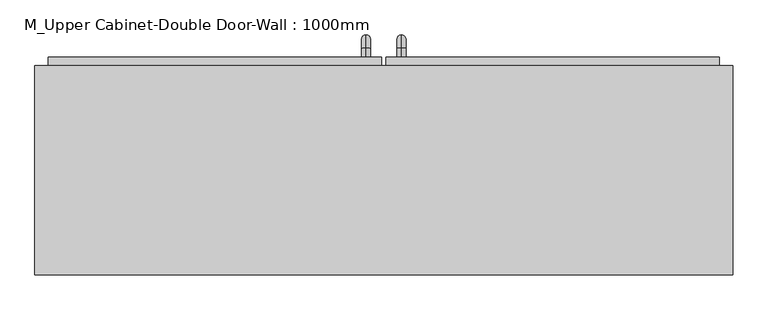
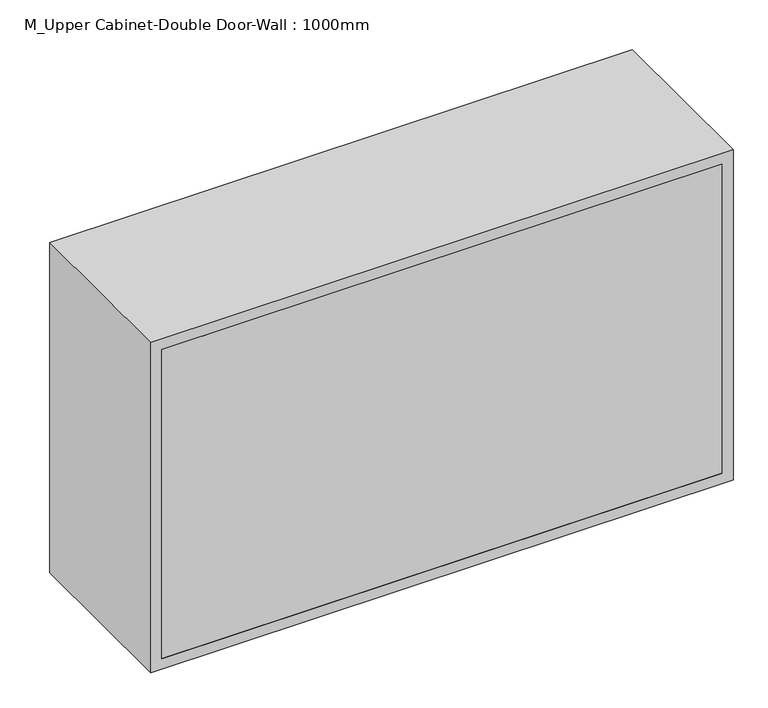
"""IFC4 building model written with IfcOpenShell, lengths in millimetres: furniture geometry, M_Upper Cabinet-Double Door-Wall : 1000mm."""

from ifc_helpers import new_model, si_unit, point, frame, origin, place, context, project, spatial, polyline, circle_curve, ellipse_curve, trimmed, outline, extrude, source, transform, mapped, element, save
from ifc_brep_helpers import plane_surface, cylinder_surface, revolved_surface, advanced_brep


def m_upper_cabinet_double_door_wall_1000mm_a8185405(model_context):
    return source(origin(), model_context, "Body", "SolidModel", [
        extrude(outline(polyline([(2000.0, -470.2288372), (1400.0, -470.2288372), (1400.0, 529.7711628), (2000.0, 529.7711628), (2000.0, -470.2288372)]), holes=[polyline([(1980.95, -451.1788372), (1980.95, 510.7211628), (1419.05, 510.7211628), (1419.05, -451.1788372), (1980.95, -451.1788372)])]), frame((0.0, 174.5, 0.0), z_axis=(0.0, 1.0, 0.0), x_axis=(0.0, 0.0, 1.0)), (0.0, 0.0, 1.0), 300.0),
        extrude(outline(polyline([(510.7211628, 174.5), (-451.1788372, 174.5), (-451.1788372, 193.55), (510.7211628, 193.55), (510.7211628, 174.5)])), frame((0.0, 0.0, 1419.05), z_axis=(0.0, 0.0, 1.0), x_axis=(1.0, 0.0, 0.0)), (0.0, 0.0, 1.0), 561.9),
        extrude(outline(polyline([(32.9461628, 487.2), (510.7211628, 487.2), (510.7211628, 455.45), (32.9461628, 455.45), (32.9461628, 487.2)])), frame((0.0, 0.0, 1419.05), z_axis=(0.0, 0.0, 1.0), x_axis=(1.0, 0.0, 0.0)), (0.0, 0.0, 1.0), 561.9),
        extrude(outline(polyline([(-451.1788372, 487.2), (26.5961628, 487.2), (26.5961628, 455.45), (-451.1788372, 455.45), (-451.1788372, 487.2)])), frame((0.0, 0.0, 1419.05), z_axis=(0.0, 0.0, 1.0), x_axis=(1.0, 0.0, 0.0)), (0.0, 0.0, 1.0), 561.9),
        advanced_brep(
        [(4.3711628, 487.2, 1546.05), (4.3711628, 487.2, 1558.75), (4.3711628, 499.9, 1546.05), (4.3711628, 499.9, 1558.75), (4.3711628, 518.95, 1539.7), (4.3711628, 506.25, 1539.7), (4.3711628, 506.25, 1463.5), (4.3711628, 518.95, 1463.5), (4.3711628, 499.9, 1444.45), (4.3711628, 499.9, 1457.15), (4.3711628, 487.2, 1457.15), (4.3711628, 487.2, 1444.45)],
        [
            (0, 1, circle_curve(frame((4.3711628, 487.2, 1552.4), z_axis=(0.0, -1.0, 0.0), x_axis=(0.0, 0.0, 1.0)), 6.35)),
            (1, 0, circle_curve(frame((4.3711628, 487.2, 1552.4), z_axis=(0.0, -1.0, 0.0), x_axis=(0.0, 0.0, 1.0)), 6.35)),
            (0, 2),
            (2, 3, circle_curve(frame((4.3711628, 499.9, 1552.4), z_axis=(0.0, -1.0, 0.0), x_axis=(0.0, 0.0, 1.0)), 6.35)),
            (3, 1),
            (3, 2, circle_curve(frame((4.3711628, 499.9, 1552.4), z_axis=(0.0, -1.0, 0.0), x_axis=(0.0, 0.0, 1.0)), 6.35)),
            (4, 3, circle_curve(frame((4.3711628, 499.9, 1539.7), z_axis=(1.0, 0.0, 0.0), x_axis=(0.0, 0.0, 1.0)), 19.05)),
            (2, 5, circle_curve(frame((4.3711628, 499.9, 1539.7), z_axis=(-1.0, 0.0, 0.0), x_axis=(0.0, 0.0, 1.0)), 6.35)),
            (5, 4, circle_curve(frame((4.3711628, 512.6, 1539.7), z_axis=(0.0, 0.0, 1.0), x_axis=(0.0, 1.0, 0.0)), 6.35)),
            (4, 5, circle_curve(frame((4.3711628, 512.6, 1539.7), z_axis=(0.0, 0.0, 1.0), x_axis=(0.0, 1.0, 0.0)), 6.35)),
            (5, 6),
            (6, 7, circle_curve(frame((4.3711628, 512.6, 1463.5), z_axis=(0.0, 0.0, 1.0), x_axis=(0.0, 1.0, 0.0)), 6.35)),
            (7, 4),
            (7, 6, circle_curve(frame((4.3711628, 512.6, 1463.5), z_axis=(0.0, 0.0, 1.0), x_axis=(0.0, 1.0, 0.0)), 6.35)),
            (8, 7, circle_curve(frame((4.3711628, 499.9, 1463.5), z_axis=(1.0, 0.0, 0.0), x_axis=(0.0, 1.0, 0.0)), 19.05)),
            (6, 9, circle_curve(frame((4.3711628, 499.9, 1463.5), z_axis=(-1.0, 0.0, 0.0), x_axis=(0.0, 1.0, 0.0)), 6.35)),
            (9, 8, circle_curve(frame((4.3711628, 499.9, 1450.8), z_axis=(0.0, 1.0, 0.0), x_axis=(0.0, 0.0, -1.0)), 6.35)),
            (8, 9, circle_curve(frame((4.3711628, 499.9, 1450.8), z_axis=(0.0, 1.0, 0.0), x_axis=(0.0, 0.0, -1.0)), 6.35)),
            (10, 11, circle_curve(frame((4.3711628, 487.2, 1450.8), z_axis=(0.0, -1.0, 0.0), x_axis=(0.0, 0.0, -1.0)), 6.35)),
            (11, 10, circle_curve(frame((4.3711628, 487.2, 1450.8), z_axis=(0.0, -1.0, 0.0), x_axis=(0.0, 0.0, -1.0)), 6.35)),
            (9, 10),
            (11, 8),
        ],
        [
            plane_surface(frame((-1.9788372, 487.2, 1552.4), z_axis=(0.0, -1.0, 0.0), x_axis=(0.0, 0.0, 1.0))),
            cylinder_surface(frame((4.3711628, 487.2, 1552.4), z_axis=(0.0, -1.0, 0.0), x_axis=(0.0, 0.0, 1.0)), 6.35),
            revolved_surface(trimmed(ellipse_curve(frame((4.3711628, 499.9, 1552.4), z_axis=(0.0, -1.0, 0.0), x_axis=(0.0, 0.0, 1.0)), 6.35, 6.35), [point((4.3711628, 499.9, 1546.05))], [point((4.3711628, 499.9, 1558.75))], True, "CARTESIAN"), (4.3711628, 499.9, 1539.7), (-1.0, 0.0, 0.0)),
            revolved_surface(trimmed(ellipse_curve(frame((4.3711628, 499.9, 1552.4), z_axis=(0.0, -1.0, 0.0), x_axis=(0.0, 0.0, 1.0)), 6.35, 6.35), [point((4.3711628, 499.9, 1558.75))], [point((4.3711628, 499.9, 1546.05))], True, "CARTESIAN"), (4.3711628, 499.9, 1539.7), (-1.0, 0.0, 0.0)),
            cylinder_surface(frame((4.3711628, 512.6, 1539.7), z_axis=(0.0, 0.0, 1.0), x_axis=(0.0, 1.0, 0.0)), 6.35),
            revolved_surface(trimmed(ellipse_curve(frame((4.3711628, 512.6, 1463.5), z_axis=(0.0, 0.0, 1.0), x_axis=(0.0, 1.0, 0.0)), 6.35, 6.35), [point((4.3711628, 506.25, 1463.5))], [point((4.3711628, 518.95, 1463.5))], True, "CARTESIAN"), (4.3711628, 499.9, 1463.5), (-1.0, 0.0, 0.0)),
            revolved_surface(trimmed(ellipse_curve(frame((4.3711628, 512.6, 1463.5), z_axis=(0.0, 0.0, 1.0), x_axis=(0.0, 1.0, 0.0)), 6.35, 6.35), [point((4.3711628, 518.95, 1463.5))], [point((4.3711628, 506.25, 1463.5))], True, "CARTESIAN"), (4.3711628, 499.9, 1463.5), (-1.0, 0.0, 0.0)),
            plane_surface(frame((-1.9788372, 487.2, 1450.8), z_axis=(0.0, -1.0, 0.0), x_axis=(0.0, 0.0, -1.0))),
            cylinder_surface(frame((4.3711628, 499.9, 1450.8), z_axis=(0.0, 1.0, 0.0), x_axis=(0.0, 0.0, -1.0)), 6.35),
        ],
        [
            (0, [[1, 2]]),
            (1, [[-1, 3, 4, 5]]),
            (1, [[-2, -5, 6, -3]]),
            (2, [[7, -4, 8, 9]]),
            (3, [[-8, -6, -7, 10]]),
            (4, [[-9, 11, 12, 13]]),
            (4, [[-10, -13, 14, -11]]),
            (5, [[15, -12, 16, 17]]),
            (6, [[-16, -14, -15, 18]]),
            (7, [[19, 20]]),
            (8, [[-17, 21, -20, 22]]),
            (8, [[-18, -22, -19, -21]]),
        ],
    ),
        advanced_brep(
        [(55.1711628, 487.2, 1546.05), (55.1711628, 487.2, 1558.75), (55.1711628, 499.9, 1546.05), (55.1711628, 499.9, 1558.75), (55.1711628, 518.95, 1539.7), (55.1711628, 506.25, 1539.7), (55.1711628, 506.25, 1463.5), (55.1711628, 518.95, 1463.5), (55.1711628, 499.9, 1444.45), (55.1711628, 499.9, 1457.15), (55.1711628, 487.2, 1457.15), (55.1711628, 487.2, 1444.45)],
        [
            (0, 1, circle_curve(frame((55.1711628, 487.2, 1552.4), z_axis=(0.0, -1.0, 0.0), x_axis=(0.0, 0.0, -1.0)), 6.35)),
            (1, 0, circle_curve(frame((55.1711628, 487.2, 1552.4), z_axis=(0.0, -1.0, 0.0), x_axis=(0.0, 0.0, -1.0)), 6.35)),
            (0, 2),
            (2, 3, circle_curve(frame((55.1711628, 499.9, 1552.4), z_axis=(0.0, -1.0, 0.0), x_axis=(0.0, 0.0, -1.0)), 6.35)),
            (3, 1),
            (3, 2, circle_curve(frame((55.1711628, 499.9, 1552.4), z_axis=(0.0, -1.0, 0.0), x_axis=(0.0, 0.0, -1.0)), 6.35)),
            (4, 3, circle_curve(frame((55.1711628, 499.9, 1539.7), z_axis=(1.0, 0.0, 0.0), x_axis=(0.0, 0.0, 1.0)), 19.05)),
            (2, 5, circle_curve(frame((55.1711628, 499.9, 1539.7), z_axis=(-1.0, 0.0, 0.0), x_axis=(0.0, 0.0, 1.0)), 6.35)),
            (5, 4, circle_curve(frame((55.1711628, 512.6, 1539.7), z_axis=(0.0, 0.0, 1.0), x_axis=(0.0, -1.0, 0.0)), 6.35)),
            (4, 5, circle_curve(frame((55.1711628, 512.6, 1539.7), z_axis=(0.0, 0.0, 1.0), x_axis=(0.0, -1.0, 0.0)), 6.35)),
            (5, 6),
            (6, 7, circle_curve(frame((55.1711628, 512.6, 1463.5), z_axis=(0.0, 0.0, 1.0), x_axis=(0.0, -1.0, 0.0)), 6.35)),
            (7, 4),
            (7, 6, circle_curve(frame((55.1711628, 512.6, 1463.5), z_axis=(0.0, 0.0, 1.0), x_axis=(0.0, -1.0, 0.0)), 6.35)),
            (8, 7, circle_curve(frame((55.1711628, 499.9, 1463.5), z_axis=(1.0, 0.0, 0.0), x_axis=(0.0, 1.0, 0.0)), 19.05)),
            (6, 9, circle_curve(frame((55.1711628, 499.9, 1463.5), z_axis=(-1.0, 0.0, 0.0), x_axis=(0.0, 1.0, 0.0)), 6.35)),
            (9, 8, circle_curve(frame((55.1711628, 499.9, 1450.8), z_axis=(0.0, 1.0, 0.0), x_axis=(0.0, 0.0, 1.0)), 6.35)),
            (8, 9, circle_curve(frame((55.1711628, 499.9, 1450.8), z_axis=(0.0, 1.0, 0.0), x_axis=(0.0, 0.0, 1.0)), 6.35)),
            (10, 11, circle_curve(frame((55.1711628, 487.2, 1450.8), z_axis=(0.0, -1.0, 0.0), x_axis=(0.0, 0.0, 1.0)), 6.35)),
            (11, 10, circle_curve(frame((55.1711628, 487.2, 1450.8), z_axis=(0.0, -1.0, 0.0), x_axis=(0.0, 0.0, 1.0)), 6.35)),
            (9, 10),
            (11, 8),
        ],
        [
            plane_surface(frame((48.8211628, 487.2, 1552.4), z_axis=(0.0, -1.0, 0.0), x_axis=(0.0, 0.0, 1.0))),
            cylinder_surface(frame((55.1711628, 487.2, 1552.4), z_axis=(0.0, -1.0, 0.0), x_axis=(0.0, 0.0, -1.0)), 6.35),
            revolved_surface(trimmed(ellipse_curve(frame((55.1711628, 499.9, 1552.4), z_axis=(0.0, -1.0, 0.0), x_axis=(0.0, 0.0, -1.0)), 6.35, 6.35), [point((55.1711628, 499.9, 1546.05))], [point((55.1711628, 499.9, 1558.75))], True, "CARTESIAN"), (55.1711628, 499.9, 1539.7), (-1.0, 0.0, 0.0)),
            revolved_surface(trimmed(ellipse_curve(frame((55.1711628, 499.9, 1552.4), z_axis=(0.0, -1.0, 0.0), x_axis=(0.0, 0.0, -1.0)), 6.35, 6.35), [point((55.1711628, 499.9, 1558.75))], [point((55.1711628, 499.9, 1546.05))], True, "CARTESIAN"), (55.1711628, 499.9, 1539.7), (-1.0, 0.0, 0.0)),
            cylinder_surface(frame((55.1711628, 512.6, 1539.7), z_axis=(0.0, 0.0, 1.0), x_axis=(0.0, -1.0, 0.0)), 6.35),
            revolved_surface(trimmed(ellipse_curve(frame((55.1711628, 512.6, 1463.5), z_axis=(0.0, 0.0, 1.0), x_axis=(0.0, -1.0, 0.0)), 6.35, 6.35), [point((55.1711628, 506.25, 1463.5))], [point((55.1711628, 518.95, 1463.5))], True, "CARTESIAN"), (55.1711628, 499.9, 1463.5), (-1.0, 0.0, 0.0)),
            revolved_surface(trimmed(ellipse_curve(frame((55.1711628, 512.6, 1463.5), z_axis=(0.0, 0.0, 1.0), x_axis=(0.0, -1.0, 0.0)), 6.35, 6.35), [point((55.1711628, 518.95, 1463.5))], [point((55.1711628, 506.25, 1463.5))], True, "CARTESIAN"), (55.1711628, 499.9, 1463.5), (-1.0, 0.0, 0.0)),
            plane_surface(frame((48.8211628, 487.2, 1450.8), z_axis=(0.0, -1.0, 0.0), x_axis=(0.0, 0.0, -1.0))),
            cylinder_surface(frame((55.1711628, 499.9, 1450.8), z_axis=(0.0, 1.0, 0.0), x_axis=(0.0, 0.0, 1.0)), 6.35),
        ],
        [
            (0, [[1, 2]]),
            (1, [[-1, 3, 4, 5]]),
            (1, [[-2, -5, 6, -3]]),
            (2, [[7, -4, 8, 9]]),
            (3, [[-8, -6, -7, 10]]),
            (4, [[-9, 11, 12, 13]]),
            (4, [[-10, -13, 14, -11]]),
            (5, [[15, -12, 16, 17]]),
            (6, [[-16, -14, -15, 18]]),
            (7, [[19, 20]]),
            (8, [[-17, 21, -20, 22]]),
            (8, [[-18, -22, -19, -21]]),
        ],
    ),
    ])


if __name__ == "__main__":
    model = new_model("IFC4")
    model_context = context("Model", 3, world=origin())
    ifc_project = project(units=[si_unit("LENGTHUNIT", "METRE", prefix="MILLI")], contexts=[model_context])
    site = spatial("IfcSite", under=ifc_project)
    building = spatial("IfcBuilding", under=site)
    placement = place(None, origin())
    m_upper_cabinet_double_door_wall_1000mm_shape = m_upper_cabinet_double_door_wall_1000mm_a8185405(model_context)
    element("IfcFurniture", 1, ObjectType="M_Upper Cabinet-Double Door-Wall : 1000mm", at=placement, inside=building, context=model_context, shape_type="MappedRepresentation", body=[
        mapped(m_upper_cabinet_double_door_wall_1000mm_shape, transform((0.0, 0.0, 0.0), x_axis=(1.0, 0.0, 0.0), y_axis=(0.0, 1.0, 0.0), z_axis=(0.0, 0.0, 1.0))),
    ])
    save(model, "model.ifc")

# Revit data of these elements
# Type "M_Upper Cabinet-Double Door-Wall : 1000mm"
#   Depth = 300 mm
#   Height = 600 mm
#   Top Of Cabinet = 2000 mm
#   Width = 1000 mm
#   Cabinet Material = none
#   Door/Drawer Material = none
#   Handle Material = Cabinets - Handles
#   Default Elevation = 0
# Element 1 (IfcFurniture, "M_Upper Cabinet-Double Door-Wall : 1000mm")
#   Materials on its faces: "Cabinets", "Cabinets - Handles"
# Materials
#   "Cabinets - Handles": class "Metal", colour RGB 57 57 57, transparency 0, Cost = 0
#   "Cabinets": class "Miscellaneous", colour RGB 249 249 249, transparency 0, Cost = 0
